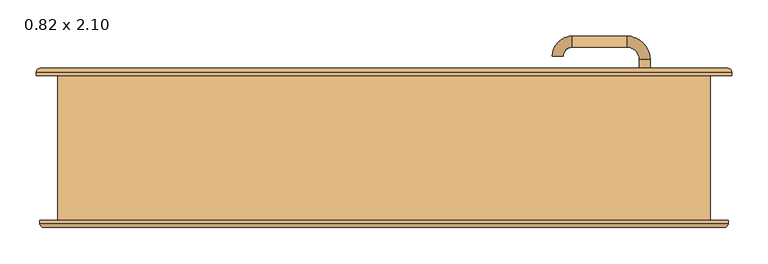
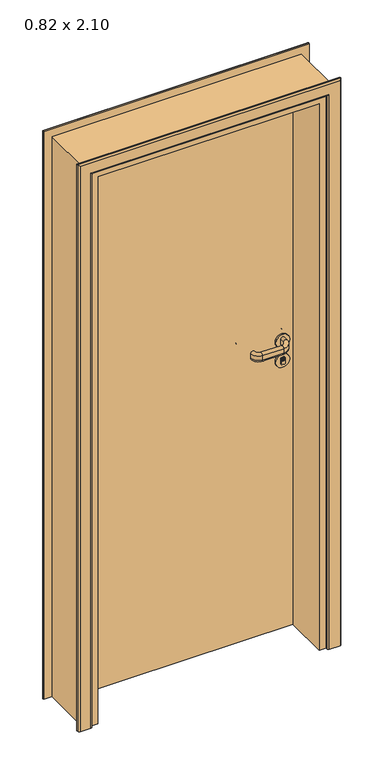
"""IFC4 building model written with IfcOpenShell, lengths in millimetres: door geometry, CC_PORTA ABRIR_1 FOLHA LISA : 0.82 x 2.10."""

from ifc_helpers import new_model, si_unit, point, frame, frame_2d, origin, origin_with_axes, place, context, project, spatial, polyline, circle_curve, ellipse_curve, trimmed, segment, composite_curve, outline, extrude, faceted_brep, source, transform, mapped, element, save
from ifc_brep_helpers import plane_surface, cylinder_surface, revolved_surface, advanced_brep


def door_0_82_x_2_10_06cf7ed5(model_context):
    return source(origin(), model_context, "Body", "SolidModel", [
        advanced_brep(
        [(352.5, 65.0, 1091.5062746), (352.5, 65.0, 1108.3826844), (367.5, 65.0, 1108.3826844), (367.5, 65.0, 1091.5062746), (367.5, 43.0, 1108.3826844), (367.5, 43.0, 1091.5062746), (352.5, 43.0, 1091.5062746), (352.5, 43.0, 1108.3826844), (335.0, 10.5, 1108.3826844), (260.0, 10.5, 1108.3826844), (260.0, 10.5, 1091.5062746), (335.0, 10.5, 1091.5062746), (335.0, 25.5, 1091.5062746), (260.0, 25.5, 1091.5062746), (260.0, 25.5, 1108.3826844), (335.0, 25.5, 1108.3826844), (247.5, 38.0, 1091.5062746), (232.5, 38.0, 1091.5062746), (232.5, 38.0, 1108.3826844), (247.5, 38.0, 1108.3826844)],
        [
            (0, 1),
            (1, 2, circle_curve(frame((360.0, 65.0, 1108.3826844), z_axis=(0.0, 1.0, 0.0), x_axis=(0.0, 0.0, 1.0)), 7.5)),
            (2, 3),
            (3, 0, circle_curve(frame((360.0, 65.0, 1091.5062746), z_axis=(0.0, 1.0, 0.0), x_axis=(0.0, 0.0, 1.0)), 7.5)),
            (2, 4),
            (4, 5),
            (5, 3),
            (0, 6),
            (6, 7),
            (7, 1),
            (8, 9),
            (9, 10),
            (10, 11),
            (11, 8),
            (12, 13),
            (13, 14),
            (14, 15),
            (15, 12),
            (5, 6, circle_curve(frame((360.0, 43.0, 1091.5062746), z_axis=(0.0, 1.0, 0.0), x_axis=(0.0, 0.0, 1.0)), 7.5)),
            (7, 4, circle_curve(frame((360.0, 43.0, 1108.3826844), z_axis=(0.0, 1.0, 0.0), x_axis=(0.0, 0.0, 1.0)), 7.5)),
            (10, 13, circle_curve(frame((260.0, 18.0, 1091.5062746), z_axis=(1.0, 0.0, 0.0), x_axis=(0.0, 0.0, 1.0)), 7.5)),
            (12, 11, circle_curve(frame((335.0, 18.0, 1091.5062746), z_axis=(-1.0, 0.0, 0.0), x_axis=(0.0, 0.0, 1.0)), 7.5)),
            (14, 9, circle_curve(frame((260.0, 18.0, 1108.3826844), z_axis=(1.0, 0.0, 0.0), x_axis=(0.0, 0.0, 1.0)), 7.5)),
            (8, 15, circle_curve(frame((335.0, 18.0, 1108.3826844), z_axis=(-1.0, 0.0, 0.0), x_axis=(0.0, 0.0, 1.0)), 7.5)),
            (12, 6, circle_curve(frame((335.0, 43.0, 1091.5062746), z_axis=(0.0, 0.0, 1.0), x_axis=(1.0, 0.0, 0.0)), 17.5)),
            (5, 11, circle_curve(frame((335.0, 43.0, 1091.5062746), z_axis=(0.0, 0.0, -1.0), x_axis=(1.0, 0.0, 0.0)), 32.5)),
            (4, 8, circle_curve(frame((335.0, 43.0, 1108.3826844), z_axis=(0.0, 0.0, -1.0), x_axis=(1.0, 0.0, 0.0)), 32.5)),
            (7, 15, circle_curve(frame((335.0, 43.0, 1108.3826844), z_axis=(0.0, 0.0, -1.0), x_axis=(1.0, 0.0, 0.0)), 17.5)),
            (16, 17, circle_curve(frame((240.0, 38.0, 1091.5062746), z_axis=(0.0, 1.0, 0.0), x_axis=(0.0, 0.0, 1.0)), 7.5)),
            (17, 18),
            (18, 19, circle_curve(frame((240.0, 38.0, 1108.3826844), z_axis=(0.0, 1.0, 0.0), x_axis=(0.0, 0.0, 1.0)), 7.5)),
            (19, 16),
            (16, 13, circle_curve(frame((260.0, 38.0, 1091.5062746), z_axis=(0.0, 0.0, 1.0), x_axis=(0.0, -1.0, 0.0)), 12.5)),
            (10, 17, circle_curve(frame((260.0, 38.0, 1091.5062746), z_axis=(0.0, 0.0, -1.0), x_axis=(0.0, -1.0, 0.0)), 27.5)),
            (9, 18, circle_curve(frame((260.0, 38.0, 1108.3826844), z_axis=(0.0, 0.0, -1.0), x_axis=(0.0, -1.0, 0.0)), 27.5)),
            (14, 19, circle_curve(frame((260.0, 38.0, 1108.3826844), z_axis=(0.0, 0.0, -1.0), x_axis=(0.0, -1.0, 0.0)), 12.5)),
        ],
        [
            plane_surface(frame((360.0, 65.0, 1099.9444795), z_axis=(0.0, 1.0, 0.0), x_axis=(0.0, 0.0, 1.0))),
            plane_surface(frame((367.5, 65.0, 1091.5062746), z_axis=(1.0, 0.0, 0.0), x_axis=(0.0, -1.0, 0.0))),
            plane_surface(frame((352.5, 65.0, 1108.3826844), z_axis=(-1.0, 0.0, 0.0), x_axis=(0.0, -1.0, 0.0))),
            plane_surface(frame((335.0, 10.5, 1091.5062746), z_axis=(0.0, -1.0, 0.0), x_axis=(-1.0, 0.0, 0.0))),
            plane_surface(frame((335.0, 25.5, 1108.3826844), z_axis=(0.0, 1.0, 0.0), x_axis=(-1.0, 0.0, 0.0))),
            cylinder_surface(frame((360.0, 65.0, 1091.5062746), z_axis=(0.0, 1.0, 0.0), x_axis=(0.0, 0.0, 1.0)), 7.5),
            cylinder_surface(frame((360.0, 65.0, 1108.3826844), z_axis=(0.0, 1.0, 0.0), x_axis=(0.0, 0.0, 1.0)), 7.5),
            cylinder_surface(frame((335.0, 18.0, 1091.5062746), z_axis=(1.0, 0.0, 0.0), x_axis=(0.0, 0.0, 1.0)), 7.5),
            cylinder_surface(frame((335.0, 18.0, 1108.3826844), z_axis=(1.0, 0.0, 0.0), x_axis=(0.0, 0.0, 1.0)), 7.5),
            revolved_surface(trimmed(ellipse_curve(frame((360.0, 43.0, 1091.5062746), z_axis=(0.0, -1.0, 0.0), x_axis=(0.0, 0.0, 1.0)), 7.5, 7.5), [point((352.5, 43.0, 1091.5062746))], [point((367.5, 43.0, 1091.5062746))], True, "CARTESIAN"), (335.0, 43.0, 1099.9444795), (0.0, 0.0, 1.0)),
            cylinder_surface(frame((335.0, 43.0, 1099.9444795), z_axis=(0.0, 0.0, 1.0), x_axis=(1.0, 0.0, 0.0)), 32.5),
            revolved_surface(trimmed(ellipse_curve(frame((360.0, 43.0, 1108.3826844), z_axis=(0.0, -1.0, 0.0), x_axis=(0.0, 0.0, 1.0)), 7.5, 7.5), [point((367.5, 43.0, 1108.3826844))], [point((352.5, 43.0, 1108.3826844))], True, "CARTESIAN"), (335.0, 43.0, 1099.9444795), (0.0, 0.0, 1.0)),
            revolved_surface(polyline([(352.5, 43.0, 1108.3826844), (352.5, 43.0, 1091.5062746)]), (335.0, 43.0, 1099.9444795), (0.0, 0.0, 1.0)),
            plane_surface(frame((240.0, 38.0, 1099.9444795), z_axis=(0.0, 1.0, 0.0), x_axis=(0.0, 0.0, 1.0))),
            revolved_surface(trimmed(ellipse_curve(frame((260.0, 18.0, 1091.5062746), z_axis=(-1.0, 0.0, 0.0), x_axis=(0.0, 0.0, 1.0)), 7.5, 7.5), [point((260.0, 25.5, 1091.5062746))], [point((260.0, 10.5, 1091.5062746))], True, "CARTESIAN"), (260.0, 38.0, 1099.9444795), (0.0, 0.0, 1.0)),
            cylinder_surface(frame((260.0, 38.0, 1099.9444795), z_axis=(0.0, 0.0, 1.0), x_axis=(0.0, -1.0, 0.0)), 27.5),
            revolved_surface(trimmed(ellipse_curve(frame((260.0, 18.0, 1108.3826844), z_axis=(-1.0, 0.0, 0.0), x_axis=(0.0, 0.0, 1.0)), 7.5, 7.5), [point((260.0, 10.5, 1108.3826844))], [point((260.0, 25.5, 1108.3826844))], True, "CARTESIAN"), (260.0, 38.0, 1099.9444795), (0.0, 0.0, 1.0)),
            revolved_surface(polyline([(260.0, 25.5, 1108.3826844), (260.0, 25.5, 1091.5062746)]), (260.0, 38.0, 1099.9444795), (0.0, 0.0, 1.0)),
        ],
        [
            (0, [[1, 2, 3, 4]]),
            (1, [[5, 6, 7, -3]]),
            (2, [[8, 9, 10, -1]]),
            (3, [[11, 12, 13, 14]]),
            (4, [[15, 16, 17, 18]]),
            (5, [[-7, 19, -8, -4]]),
            (6, [[-10, 20, -5, -2]]),
            (7, [[-13, 21, -15, 22]]),
            (8, [[-17, 23, -11, 24]]),
            (9, [[-22, 25, -19, 26]]),
            (10, [[-14, -26, -6, 27]]),
            (11, [[-24, -27, -20, 28]]),
            (12, [[-18, -28, -9, -25]]),
            (13, [[29, 30, 31, 32]]),
            (14, [[-29, 33, -21, 34]]),
            (15, [[-30, -34, -12, 35]]),
            (16, [[-31, -35, -23, 36]]),
            (17, [[-32, -36, -16, -33]]),
        ],
    ),
        extrude(outline(polyline([(361.0, 65.0), (361.0, 55.9), (359.0, 55.9), (359.0, 65.0), (361.0, 65.0)])), frame((0.0, 0.0, 1027.9555433), z_axis=(0.0, 0.0, 1.0), x_axis=(1.0, 0.0, 0.0)), (0.0, 0.0, 1.0), 7.8071257),
        extrude(outline(composite_curve([segment(trimmed(circle_curve(frame_2d((1031.5611613, 360.0)), 5.0), [point((1036.5611613, 360.0))], [point((1026.5611613, 360.0))], False, "CARTESIAN"), True, "CONTINUOUS"), segment(trimmed(circle_curve(frame_2d((1031.5611613, 360.0)), 5.0), [point((1026.5611613, 360.0))], [point((1036.5611613, 360.0))], False, "CARTESIAN"), True, "CONTINUOUS")], self_intersect=False), holes=[polyline([(1035.7626689, 361.0), (1027.9555433, 361.0), (1027.9555433, 359.0), (1035.7626689, 359.0), (1035.7626689, 361.0)])]), frame((0.0, 55.0, 0.0), z_axis=(0.0, 1.0, 0.0), x_axis=(0.0, 0.0, 1.0)), (0.0, 0.0, 1.0), 10.0),
        extrude(outline(composite_curve([segment(polyline([(1033.4817325, 352.5), (1016.4817325, 352.5)]), True, "CONTINUOUS"), segment(trimmed(circle_curve(frame_2d((1016.4817325, 356.5)), 4.0), [point((1016.4817325, 352.5))], [point((1012.4817325, 356.5))], False, "CARTESIAN"), True, "CONTINUOUS"), segment(polyline([(1012.4817325, 356.5), (1012.4817325, 363.5)]), True, "CONTINUOUS"), segment(trimmed(circle_curve(frame_2d((1016.4817325, 363.5)), 4.0), [point((1012.4817325, 363.5))], [point((1016.4817325, 367.5))], False, "CARTESIAN"), True, "CONTINUOUS"), segment(polyline([(1016.4817325, 367.5), (1033.4817325, 367.5)]), True, "CONTINUOUS"), segment(trimmed(circle_curve(frame_2d((1033.4817325, 363.5)), 4.0), [point((1033.4817325, 367.5))], [point((1037.4817325, 363.5))], False, "CARTESIAN"), True, "CONTINUOUS"), segment(polyline([(1037.4817325, 363.5), (1037.4817325, 356.5)]), True, "CONTINUOUS"), segment(trimmed(circle_curve(frame_2d((1033.4817325, 356.5)), 4.0), [point((1037.4817325, 356.5))], [point((1033.4817325, 352.5))], False, "CARTESIAN"), True, "CONTINUOUS")], self_intersect=False)), frame((0.0, 56.0, 0.0), z_axis=(0.0, 1.0, 0.0), x_axis=(0.0, 0.0, 1.0)), (0.0, 0.0, 1.0), 9.0),
        extrude(outline(composite_curve([segment(trimmed(circle_curve(frame_2d((1099.9444795, 360.0)), 25.0), [point((1124.9444795, 360.0))], [point((1074.9444795, 360.0))], False, "CARTESIAN"), True, "CONTINUOUS"), segment(trimmed(circle_curve(frame_2d((1099.9444795, 360.0)), 25.0), [point((1074.9444795, 360.0))], [point((1124.9444795, 360.0))], False, "CARTESIAN"), True, "CONTINUOUS")], self_intersect=False)), frame((0.0, 59.0, 0.0), z_axis=(0.0, 1.0, 0.0), x_axis=(0.0, 0.0, 1.0)), (0.0, 0.0, 1.0), 6.0),
        extrude(outline(composite_curve([segment(trimmed(circle_curve(frame_2d((1024.9444795, 360.0)), 25.0), [point((1049.9444795, 360.0))], [point((999.9444795, 360.0))], False, "CARTESIAN"), True, "CONTINUOUS"), segment(trimmed(circle_curve(frame_2d((1024.9444795, 360.0)), 25.0), [point((999.9444795, 360.0))], [point((1049.9444795, 360.0))], False, "CARTESIAN"), True, "CONTINUOUS")], self_intersect=False), holes=[composite_curve([segment(trimmed(circle_curve(frame_2d((1033.4817325, 363.5)), 4.0), [point((1037.4817325, 363.5))], [point((1033.4817325, 367.5))], True, "CARTESIAN"), True, "CONTINUOUS"), segment(polyline([(1033.4817325, 367.5), (1016.4817325, 367.5)]), True, "CONTINUOUS"), segment(trimmed(circle_curve(frame_2d((1016.4817325, 363.5)), 4.0), [point((1016.4817325, 367.5))], [point((1012.4817325, 363.5))], True, "CARTESIAN"), True, "CONTINUOUS"), segment(polyline([(1012.4817325, 363.5), (1012.4817325, 356.5)]), True, "CONTINUOUS"), segment(trimmed(circle_curve(frame_2d((1016.4817325, 356.5)), 4.0), [point((1012.4817325, 356.5))], [point((1016.4817325, 352.5))], True, "CARTESIAN"), True, "CONTINUOUS"), segment(polyline([(1016.4817325, 352.5), (1033.4817325, 352.5)]), True, "CONTINUOUS"), segment(trimmed(circle_curve(frame_2d((1033.4817325, 356.5)), 4.0), [point((1033.4817325, 352.5))], [point((1037.4817325, 356.5))], True, "CARTESIAN"), True, "CONTINUOUS"), segment(polyline([(1037.4817325, 356.5), (1037.4817325, 363.5)]), True, "CONTINUOUS")], self_intersect=False)]), frame((0.0, 59.0, 0.0), z_axis=(0.0, 1.0, 0.0), x_axis=(0.0, 0.0, 1.0)), (0.0, 0.0, 1.0), 6.0),
        extrude(outline(polyline([(361.0, 109.1), (361.0, 100.0), (359.0, 100.0), (359.0, 109.1), (361.0, 109.1)])), frame((0.0, 0.0, 1027.9555433), z_axis=(0.0, 0.0, 1.0), x_axis=(1.0, 0.0, 0.0)), (0.0, 0.0, 1.0), 7.8071257),
        advanced_brep(
        [(360.0, 110.0, 1036.5611613), (360.0, 110.0, 1026.5611613), (361.0, 110.0, 1035.7626689), (359.0, 110.0, 1035.7626689), (359.0, 110.0, 1027.9555433), (361.0, 110.0, 1027.9555433), (360.0, 100.0, 1049.9444795), (360.0, 100.0, 999.9444795), (360.0, 109.0, 1026.5611613), (360.0, 109.0, 1036.5611613), (361.0, 109.0, 1027.9555433), (361.0, 109.0, 1035.7626689), (359.0, 109.0, 1027.9555433), (359.0, 109.0, 1035.7626689), (352.5, 109.0, 1033.4817325), (356.5, 109.0, 1037.4817325), (363.5, 109.0, 1037.4817325), (367.5, 109.0, 1033.4817325), (367.5, 109.0, 1016.4817325), (363.5, 109.0, 1012.4817325), (356.5, 109.0, 1012.4817325), (352.5, 109.0, 1016.4817325), (352.5, 106.0, 1016.4817325), (352.5, 106.0, 1033.4817325), (356.5, 106.0, 1012.4817325), (363.5, 106.0, 1012.4817325), (367.5, 106.0, 1016.4817325), (367.5, 106.0, 1033.4817325), (363.5, 106.0, 1037.4817325), (356.5, 106.0, 1037.4817325), (360.0, 106.0, 1049.9444795), (360.0, 106.0, 999.9444795)],
        [
            (0, 1, circle_curve(frame((360.0, 110.0, 1031.5611613), z_axis=(0.0, 1.0, 0.0), x_axis=(0.0, 0.0, -1.0)), 5.0)),
            (1, 0, circle_curve(frame((360.0, 110.0, 1031.5611613), z_axis=(0.0, 1.0, 0.0), x_axis=(0.0, 0.0, -1.0)), 5.0)),
            (2, 3),
            (3, 4),
            (4, 5),
            (5, 2),
            (6, 7, circle_curve(frame((360.0, 100.0, 1024.9444795), z_axis=(0.0, -1.0, 0.0), x_axis=(0.0, 0.0, -1.0)), 25.0)),
            (7, 6, circle_curve(frame((360.0, 100.0, 1024.9444795), z_axis=(0.0, -1.0, 0.0), x_axis=(0.0, 0.0, -1.0)), 25.0)),
            (1, 8),
            (8, 9, circle_curve(frame((360.0, 109.0, 1031.5611613), z_axis=(0.0, 1.0, 0.0), x_axis=(0.0, 0.0, -1.0)), 5.0)),
            (9, 0),
            (9, 8, circle_curve(frame((360.0, 109.0, 1031.5611613), z_axis=(0.0, 1.0, 0.0), x_axis=(0.0, 0.0, -1.0)), 5.0)),
            (5, 10),
            (10, 11),
            (11, 2),
            (4, 12),
            (12, 10),
            (3, 13),
            (13, 12),
            (11, 13),
            (14, 15, circle_curve(frame((356.5, 109.0, 1033.4817325), z_axis=(0.0, 1.0, 0.0), x_axis=(0.0, 0.0, -1.0)), 4.0)),
            (15, 16),
            (16, 17, circle_curve(frame((363.5, 109.0, 1033.4817325), z_axis=(0.0, 1.0, 0.0), x_axis=(0.0, 0.0, -1.0)), 4.0)),
            (17, 18),
            (18, 19, circle_curve(frame((363.5, 109.0, 1016.4817325), z_axis=(0.0, 1.0, 0.0), x_axis=(0.0, 0.0, -1.0)), 4.0)),
            (19, 20),
            (20, 21, circle_curve(frame((356.5, 109.0, 1016.4817325), z_axis=(0.0, 1.0, 0.0), x_axis=(0.0, 0.0, -1.0)), 4.0)),
            (21, 14),
            (21, 22),
            (22, 23),
            (23, 14),
            (20, 24),
            (24, 22, circle_curve(frame((356.5, 106.0, 1016.4817325), z_axis=(0.0, 1.0, 0.0), x_axis=(0.0, 0.0, -1.0)), 4.0)),
            (19, 25),
            (25, 24),
            (18, 26),
            (26, 25, circle_curve(frame((363.5, 106.0, 1016.4817325), z_axis=(0.0, 1.0, 0.0), x_axis=(0.0, 0.0, -1.0)), 4.0)),
            (17, 27),
            (27, 26),
            (16, 28),
            (28, 27, circle_curve(frame((363.5, 106.0, 1033.4817325), z_axis=(0.0, 1.0, 0.0), x_axis=(0.0, 0.0, -1.0)), 4.0)),
            (15, 29),
            (29, 28),
            (23, 29, circle_curve(frame((356.5, 106.0, 1033.4817325), z_axis=(0.0, 1.0, 0.0), x_axis=(0.0, 0.0, -1.0)), 4.0)),
            (30, 31, circle_curve(frame((360.0, 106.0, 1024.9444795), z_axis=(0.0, 1.0, 0.0), x_axis=(0.0, 0.0, -1.0)), 25.0)),
            (31, 30, circle_curve(frame((360.0, 106.0, 1024.9444795), z_axis=(0.0, 1.0, 0.0), x_axis=(0.0, 0.0, -1.0)), 25.0)),
            (31, 7),
            (6, 30),
        ],
        [
            plane_surface(frame((360.0, 110.0, 1026.5611613), z_axis=(0.0, 1.0, 0.0), x_axis=(1.0, 0.0, 0.0))),
            plane_surface(frame((360.0, 100.0, 1026.5611613), z_axis=(0.0, -1.0, 0.0), x_axis=(-1.0, 0.0, 0.0))),
            cylinder_surface(frame((360.0, 100.0, 1031.5611613), z_axis=(0.0, 1.0, 0.0), x_axis=(0.0, 0.0, -1.0)), 5.0),
            plane_surface(frame((361.0, 110.0, 1035.7626689), z_axis=(-1.0, 0.0, 0.0), x_axis=(0.0, -1.0, 0.0))),
            plane_surface(frame((361.0, 110.0, 1027.9555433), z_axis=(0.0, 0.0, 1.0), x_axis=(0.0, -1.0, 0.0))),
            plane_surface(frame((359.0, 110.0, 1027.9555433), z_axis=(1.0, 0.0, 0.0), x_axis=(0.0, -1.0, 0.0))),
            plane_surface(frame((359.0, 110.0, 1035.7626689), z_axis=(0.0, 0.0, -1.0), x_axis=(0.0, -1.0, 0.0))),
            plane_surface(frame((352.5, 109.0, 1016.4817325), z_axis=(0.0, 1.0, 0.0), x_axis=(0.0, 0.0, -1.0))),
            plane_surface(frame((352.5, 109.0, 1033.4817325), z_axis=(-1.0, 0.0, 0.0), x_axis=(0.0, -1.0, 0.0))),
            cylinder_surface(frame((356.5, 100.0, 1016.4817325), z_axis=(0.0, 1.0, 0.0), x_axis=(0.0, 0.0, -1.0)), 4.0),
            plane_surface(frame((356.5, 109.0, 1012.4817325), z_axis=(0.0, 0.0, -1.0), x_axis=(0.0, -1.0, 0.0))),
            cylinder_surface(frame((363.5, 100.0, 1016.4817325), z_axis=(0.0, 1.0, 0.0), x_axis=(0.0, 0.0, -1.0)), 4.0),
            plane_surface(frame((367.5, 109.0, 1016.4817325), z_axis=(1.0, 0.0, 0.0), x_axis=(0.0, -1.0, 0.0))),
            cylinder_surface(frame((363.5, 100.0, 1033.4817325), z_axis=(0.0, 1.0, 0.0), x_axis=(0.0, 0.0, -1.0)), 4.0),
            plane_surface(frame((363.5, 109.0, 1037.4817325), z_axis=(0.0, 0.0, 1.0), x_axis=(0.0, -1.0, 0.0))),
            cylinder_surface(frame((356.5, 100.0, 1033.4817325), z_axis=(0.0, 1.0, 0.0), x_axis=(0.0, 0.0, -1.0)), 4.0),
            plane_surface(frame((360.0, 106.0, 1074.9444795), z_axis=(0.0, 1.0, 0.0), x_axis=(1.0, 0.0, 0.0))),
            cylinder_surface(frame((360.0, 100.0, 1024.9444795), z_axis=(0.0, 1.0, 0.0), x_axis=(0.0, 0.0, -1.0)), 25.0),
        ],
        [
            (0, [[1, 2], [3, 4, 5, 6]]),
            (1, [[7, 8]]),
            (2, [[9, 10, 11, -2]]),
            (2, [[-11, 12, -9, -1]]),
            (3, [[13, 14, 15, -6]]),
            (4, [[16, 17, -13, -5]]),
            (5, [[18, 19, -16, -4]]),
            (6, [[-15, 20, -18, -3]]),
            (7, [[-17, -19, -20, -14]]),
            (7, [[21, 22, 23, 24, 25, 26, 27, 28], [-12, -10]]),
            (8, [[29, 30, 31, -28]]),
            (9, [[32, 33, -29, -27]]),
            (10, [[34, 35, -32, -26]]),
            (11, [[36, 37, -34, -25]]),
            (12, [[38, 39, -36, -24]]),
            (13, [[40, 41, -38, -23]]),
            (14, [[42, 43, -40, -22]]),
            (15, [[-31, 44, -42, -21]]),
            (16, [[45, 46], [-33, -35, -37, -39, -41, -43, -44, -30]]),
            (17, [[47, -7, 48, -46]]),
            (17, [[-48, -8, -47, -45]]),
        ],
    ),
        advanced_brep(
        [(360.0, 100.0, 1124.9444795), (360.0, 100.0, 1074.9444795), (360.0, 106.0, 1124.9444795), (360.0, 106.0, 1074.9444795)],
        [
            (0, 1, circle_curve(frame((360.0, 100.0, 1099.9444795), z_axis=(0.0, -1.0, 0.0), x_axis=(0.0, 0.0, -1.0)), 25.0)),
            (1, 0, circle_curve(frame((360.0, 100.0, 1099.9444795), z_axis=(0.0, -1.0, 0.0), x_axis=(0.0, 0.0, -1.0)), 25.0)),
            (2, 3, circle_curve(frame((360.0, 106.0, 1099.9444795), z_axis=(0.0, 1.0, 0.0), x_axis=(0.0, 0.0, -1.0)), 25.0)),
            (3, 2, circle_curve(frame((360.0, 106.0, 1099.9444795), z_axis=(0.0, 1.0, 0.0), x_axis=(0.0, 0.0, -1.0)), 25.0)),
            (3, 1),
            (0, 2),
        ],
        [
            plane_surface(frame((360.0, 100.0, 1026.5611613), z_axis=(0.0, -1.0, 0.0), x_axis=(-1.0, 0.0, 0.0))),
            plane_surface(frame((360.0, 106.0, 1074.9444795), z_axis=(0.0, 1.0, 0.0), x_axis=(1.0, 0.0, 0.0))),
            cylinder_surface(frame((360.0, 100.0, 1099.9444795), z_axis=(0.0, 1.0, 0.0), x_axis=(0.0, 0.0, -1.0)), 25.0),
        ],
        [
            (0, [[1, 2]]),
            (1, [[3, 4]]),
            (2, [[5, -1, 6, -4]]),
            (2, [[-6, -2, -5, -3]]),
        ],
    ),
        advanced_brep(
        [(352.5, 100.0, 1108.4382049), (352.5, 100.0, 1091.5617951), (367.5, 100.0, 1091.5617951), (367.5, 100.0, 1108.4382049), (367.5, 122.0, 1091.5617951), (367.5, 122.0, 1108.4382049), (352.5, 122.0, 1108.4382049), (352.5, 122.0, 1091.5617951), (335.0, 154.5, 1091.5617951), (260.0, 154.5, 1091.5617951), (260.0, 154.5, 1108.4382049), (335.0, 154.5, 1108.4382049), (335.0, 139.5, 1108.4382049), (260.0, 139.5, 1108.4382049), (260.0, 139.5, 1091.5617951), (335.0, 139.5, 1091.5617951), (247.5, 127.0, 1108.4382049), (232.5, 127.0, 1108.4382049), (232.5, 127.0, 1091.5617951), (247.5, 127.0, 1091.5617951)],
        [
            (0, 1),
            (1, 2, circle_curve(frame((360.0, 100.0, 1091.5617951), z_axis=(0.0, -1.0, 0.0), x_axis=(-1.0, 0.0, 0.0)), 7.5)),
            (2, 3),
            (3, 0, circle_curve(frame((360.0, 100.0, 1108.4382049), z_axis=(0.0, -1.0, 0.0), x_axis=(-1.0, 0.0, 0.0)), 7.5)),
            (2, 4),
            (4, 5),
            (5, 3),
            (0, 6),
            (6, 7),
            (7, 1),
            (8, 9),
            (9, 10),
            (10, 11),
            (11, 8),
            (12, 13),
            (13, 14),
            (14, 15),
            (15, 12),
            (5, 6, circle_curve(frame((360.0, 122.0, 1108.4382049), z_axis=(0.0, -1.0, 0.0), x_axis=(-1.0, 0.0, 0.0)), 7.5)),
            (7, 4, circle_curve(frame((360.0, 122.0, 1091.5617951), z_axis=(0.0, -1.0, 0.0), x_axis=(-1.0, 0.0, 0.0)), 7.5)),
            (10, 13, circle_curve(frame((260.0, 147.0, 1108.4382049), z_axis=(1.0, 0.0, 0.0), x_axis=(0.0, -1.0, 0.0)), 7.5)),
            (12, 11, circle_curve(frame((335.0, 147.0, 1108.4382049), z_axis=(-1.0, 0.0, 0.0), x_axis=(0.0, -1.0, 0.0)), 7.5)),
            (14, 9, circle_curve(frame((260.0, 147.0, 1091.5617951), z_axis=(1.0, 0.0, 0.0), x_axis=(0.0, -1.0, 0.0)), 7.5)),
            (8, 15, circle_curve(frame((335.0, 147.0, 1091.5617951), z_axis=(-1.0, 0.0, 0.0), x_axis=(0.0, -1.0, 0.0)), 7.5)),
            (12, 6, circle_curve(frame((335.0, 122.0, 1108.4382049), z_axis=(0.0, 0.0, -1.0), x_axis=(1.0, 0.0, 0.0)), 17.5)),
            (5, 11, circle_curve(frame((335.0, 122.0, 1108.4382049), z_axis=(0.0, 0.0, 1.0), x_axis=(1.0, 0.0, 0.0)), 32.5)),
            (4, 8, circle_curve(frame((335.0, 122.0, 1091.5617951), z_axis=(0.0, 0.0, 1.0), x_axis=(1.0, 0.0, 0.0)), 32.5)),
            (7, 15, circle_curve(frame((335.0, 122.0, 1091.5617951), z_axis=(0.0, 0.0, 1.0), x_axis=(1.0, 0.0, 0.0)), 17.5)),
            (16, 17, circle_curve(frame((240.0, 127.0, 1108.4382049), z_axis=(0.0, -1.0, 0.0), x_axis=(1.0, 0.0, 0.0)), 7.5)),
            (17, 18),
            (18, 19, circle_curve(frame((240.0, 127.0, 1091.5617951), z_axis=(0.0, -1.0, 0.0), x_axis=(1.0, 0.0, 0.0)), 7.5)),
            (19, 16),
            (16, 13, circle_curve(frame((260.0, 127.0, 1108.4382049), z_axis=(0.0, 0.0, -1.0), x_axis=(0.0, 1.0, 0.0)), 12.5)),
            (10, 17, circle_curve(frame((260.0, 127.0, 1108.4382049), z_axis=(0.0, 0.0, 1.0), x_axis=(0.0, 1.0, 0.0)), 27.5)),
            (9, 18, circle_curve(frame((260.0, 127.0, 1091.5617951), z_axis=(0.0, 0.0, 1.0), x_axis=(0.0, 1.0, 0.0)), 27.5)),
            (14, 19, circle_curve(frame((260.0, 127.0, 1091.5617951), z_axis=(0.0, 0.0, 1.0), x_axis=(0.0, 1.0, 0.0)), 12.5)),
        ],
        [
            plane_surface(frame((360.0, 100.0, 1100.0), z_axis=(0.0, -1.0, 0.0), x_axis=(0.0, 0.0, -1.0))),
            plane_surface(frame((367.5, 100.0, 1108.4382049), z_axis=(1.0, 0.0, 0.0), x_axis=(0.0, 1.0, 0.0))),
            plane_surface(frame((352.5, 100.0, 1091.5617951), z_axis=(-1.0, 0.0, 0.0), x_axis=(0.0, 1.0, 0.0))),
            plane_surface(frame((335.0, 154.5, 1108.4382049), z_axis=(0.0, 1.0, 0.0), x_axis=(-1.0, 0.0, 0.0))),
            plane_surface(frame((335.0, 139.5, 1091.5617951), z_axis=(0.0, -1.0, 0.0), x_axis=(-1.0, 0.0, 0.0))),
            cylinder_surface(frame((360.0, 100.0, 1108.4382049), z_axis=(0.0, -1.0, 0.0), x_axis=(-1.0, 0.0, 0.0)), 7.5),
            cylinder_surface(frame((360.0, 100.0, 1091.5617951), z_axis=(0.0, -1.0, 0.0), x_axis=(-1.0, 0.0, 0.0)), 7.5),
            cylinder_surface(frame((335.0, 147.0, 1108.4382049), z_axis=(1.0, 0.0, 0.0), x_axis=(0.0, -1.0, 0.0)), 7.5),
            cylinder_surface(frame((335.0, 147.0, 1091.5617951), z_axis=(1.0, 0.0, 0.0), x_axis=(0.0, -1.0, 0.0)), 7.5),
            revolved_surface(trimmed(ellipse_curve(frame((360.0, 122.0, 1108.4382049), z_axis=(0.0, 1.0, 0.0), x_axis=(-1.0, 0.0, 0.0)), 7.5, 7.5), [point((352.5, 122.0, 1108.4382049))], [point((367.5, 122.0, 1108.4382049))], True, "CARTESIAN"), (335.0, 122.0, 1100.0), (0.0, 0.0, -1.0)),
            cylinder_surface(frame((335.0, 122.0, 1100.0), z_axis=(0.0, 0.0, -1.0), x_axis=(1.0, 0.0, 0.0)), 32.5),
            revolved_surface(trimmed(ellipse_curve(frame((360.0, 122.0, 1091.5617951), z_axis=(0.0, 1.0, 0.0), x_axis=(-1.0, 0.0, 0.0)), 7.5, 7.5), [point((367.5, 122.0, 1091.5617951))], [point((352.5, 122.0, 1091.5617951))], True, "CARTESIAN"), (335.0, 122.0, 1100.0), (0.0, 0.0, -1.0)),
            revolved_surface(polyline([(352.5, 122.0, 1091.5617951), (352.5, 122.0, 1108.4382049)]), (335.0, 122.0, 1100.0), (0.0, 0.0, -1.0)),
            plane_surface(frame((240.0, 127.0, 1100.0), z_axis=(0.0, -1.0, 0.0), x_axis=(0.0, 0.0, -1.0))),
            revolved_surface(trimmed(ellipse_curve(frame((260.0, 147.0, 1108.4382049), z_axis=(-1.0, 0.0, 0.0), x_axis=(0.0, -1.0, 0.0)), 7.5, 7.5), [point((260.0, 139.5, 1108.4382049))], [point((260.0, 154.5, 1108.4382049))], True, "CARTESIAN"), (260.0, 127.0, 1100.0), (0.0, 0.0, -1.0)),
            cylinder_surface(frame((260.0, 127.0, 1100.0), z_axis=(0.0, 0.0, -1.0), x_axis=(0.0, 1.0, 0.0)), 27.5),
            revolved_surface(trimmed(ellipse_curve(frame((260.0, 147.0, 1091.5617951), z_axis=(-1.0, 0.0, 0.0), x_axis=(0.0, -1.0, 0.0)), 7.5, 7.5), [point((260.0, 154.5, 1091.5617951))], [point((260.0, 139.5, 1091.5617951))], True, "CARTESIAN"), (260.0, 127.0, 1100.0), (0.0, 0.0, -1.0)),
            revolved_surface(polyline([(260.0, 139.5, 1091.5617951), (260.0, 139.5, 1108.4382049)]), (260.0, 127.0, 1100.0), (0.0, 0.0, -1.0)),
        ],
        [
            (0, [[1, 2, 3, 4]]),
            (1, [[5, 6, 7, -3]]),
            (2, [[8, 9, 10, -1]]),
            (3, [[11, 12, 13, 14]]),
            (4, [[15, 16, 17, 18]]),
            (5, [[-7, 19, -8, -4]]),
            (6, [[-10, 20, -5, -2]]),
            (7, [[-13, 21, -15, 22]]),
            (8, [[-17, 23, -11, 24]]),
            (9, [[-22, 25, -19, 26]]),
            (10, [[-14, -26, -6, 27]]),
            (11, [[-24, -27, -20, 28]]),
            (12, [[-18, -28, -9, -25]]),
            (13, [[29, 30, 31, 32]]),
            (14, [[-29, 33, -21, 34]]),
            (15, [[-30, -34, -12, 35]]),
            (16, [[-31, -35, -23, 36]]),
            (17, [[-32, -36, -16, -33]]),
        ],
    ),
        extrude(outline(polyline([(410.0, 100.0), (410.0, 65.0), (-410.0, 65.0), (-410.0, 100.0), (410.0, 100.0)])), origin_with_axes(), (0.0, 0.0, 1.0), 2100.0),
        advanced_brep(
        [(-430.5, -110.0, 0.0), (-469.500573, -110.0, 0.0), (-475.0, -104.500573, 0.0), (-475.0, -100.0, 0.0), (-425.0, -100.0, 0.0), (-425.0, -104.5, 0.0), (-425.0, -104.5, 2115.0), (-430.5, -110.0, 2120.5), (-425.0, -100.0, 2115.0), (-475.0, -100.0, 2165.0), (475.0, -100.0, 2165.0), (475.0, -100.0, 0.0), (425.0, -100.0, 0.0), (425.0, -100.0, 2115.0), (-475.0, -104.500573, 2165.0), (-469.500573, -110.0, 2159.500573), (430.5, -110.0, 2120.5), (430.5, -110.0, 0.0), (469.500573, -110.0, 0.0), (469.500573, -110.0, 2159.500573), (425.0, -104.5, 0.0), (425.0, -104.5, 2115.0), (475.0, -104.500573, 0.0), (475.0, -104.500573, 2165.0)],
        [
            (0, 1),
            (1, 2, circle_curve(frame((-469.500573, -104.500573, 0.0), z_axis=(0.0, 0.0, -1.0), x_axis=(0.0, -1.0, 0.0)), 5.499427)),
            (2, 3),
            (3, 4),
            (4, 5),
            (5, 0, circle_curve(frame((-430.5, -104.5, 0.0), z_axis=(0.0, 0.0, -1.0), x_axis=(0.0, -1.0, 0.0)), 5.5)),
            (5, 6),
            (6, 7, ellipse_curve(frame((-430.5, -104.5, 2120.5), z_axis=(-0.7071067811865475, 0.0, -0.7071067811865475), x_axis=(0.7071067811865474, 0.0, -0.7071067811865476)), 7.7781746, 5.5)),
            (7, 0),
            (4, 8),
            (8, 6),
            (3, 9),
            (9, 10),
            (10, 11),
            (11, 12),
            (12, 13),
            (13, 8),
            (2, 14),
            (14, 9),
            (1, 15),
            (15, 14, ellipse_curve(frame((-469.500573, -104.500573, 2159.500573), z_axis=(-0.7071067811865475, 0.0, -0.7071067811865475), x_axis=(0.7071067811865474, 0.0, -0.7071067811865476)), 7.7773642, 5.499427)),
            (7, 16),
            (16, 17),
            (17, 18),
            (18, 19),
            (19, 15),
            (12, 20),
            (20, 21),
            (21, 13),
            (17, 20, circle_curve(frame((430.5, -104.5, 0.0), z_axis=(0.0, 0.0, -1.0), x_axis=(0.0, -1.0, 0.0)), 5.5)),
            (11, 22),
            (22, 18, circle_curve(frame((469.500573, -104.500573, 0.0), z_axis=(0.0, 0.0, -1.0), x_axis=(0.0, -1.0, 0.0)), 5.499427)),
            (23, 22),
            (10, 23),
            (23, 19, ellipse_curve(frame((469.500573, -104.500573, 2159.500573), z_axis=(0.7071067811865475, 0.0, -0.7071067811865475), x_axis=(0.7071067811865474, 0.0, 0.7071067811865476)), 7.7773642, 5.499427)),
            (16, 21, ellipse_curve(frame((430.5, -104.5, 2120.5), z_axis=(0.7071067811865475, 0.0, -0.7071067811865475), x_axis=(0.7071067811865474, 0.0, 0.7071067811865476)), 7.7781746, 5.5)),
            (6, 21),
            (14, 23),
        ],
        [
            plane_surface(frame((-450.0, -100.0, 0.0), z_axis=(0.0, 0.0, -1.0), x_axis=(-1.0, 0.0, 0.0))),
            cylinder_surface(frame((-430.5, -104.5, 0.0), z_axis=(0.0, 0.0, -1.0), x_axis=(0.0, -1.0, 0.0)), 5.5),
            plane_surface(frame((-425.0, -104.5, 0.0), z_axis=(1.0, 0.0, 0.0), x_axis=(0.0, 0.0, 1.0))),
            plane_surface(frame((-425.0, -100.0, 0.0), z_axis=(0.0, 1.0, 0.0), x_axis=(0.0, 0.0, 1.0))),
            plane_surface(frame((-475.0, -100.0, 0.0), z_axis=(-1.0, 0.0, 0.0), x_axis=(0.0, 0.0, 1.0))),
            cylinder_surface(frame((-469.500573, -104.500573, 0.0), z_axis=(0.0, 0.0, -1.0), x_axis=(0.0, -1.0, 0.0)), 5.499427),
            plane_surface(frame((-469.500573, -110.0, 0.0), z_axis=(0.0, -1.0, 0.0), x_axis=(0.0, 0.0, 1.0))),
            plane_surface(frame((425.0, -104.5, 2115.0), z_axis=(-1.0, 0.0, 0.0), x_axis=(0.0, 0.0, -1.0))),
            plane_surface(frame((450.0, -100.0, 0.0), z_axis=(0.0, 0.0, -1.0), x_axis=(1.0, 0.0, 0.0))),
            plane_surface(frame((475.0, -100.0, 2165.0), z_axis=(1.0, 0.0, 0.0), x_axis=(0.0, 0.0, -1.0))),
            cylinder_surface(frame((469.500573, -104.500573, 2140.0), z_axis=(0.0, 0.0, 1.0), x_axis=(0.0, -1.0, 0.0)), 5.499427),
            cylinder_surface(frame((430.5, -104.5, 2140.0), z_axis=(0.0, 0.0, 1.0), x_axis=(0.0, -1.0, 0.0)), 5.5),
            cylinder_surface(frame((-450.0, -104.5, 2120.5), z_axis=(-1.0, 0.0, 0.0), x_axis=(0.0, -1.0, 0.0)), 5.5),
            plane_surface(frame((-425.0, -104.5, 2115.0), z_axis=(0.0, 0.0, -1.0), x_axis=(1.0, 0.0, 0.0))),
            plane_surface(frame((-475.0, -100.0, 2165.0), z_axis=(0.0, 0.0, 1.0), x_axis=(1.0, 0.0, 0.0))),
            cylinder_surface(frame((-450.0, -104.500573, 2159.500573), z_axis=(-1.0, 0.0, 0.0), x_axis=(0.0, -1.0, 0.0)), 5.499427),
        ],
        [
            (0, [[1, 2, 3, 4, 5, 6]]),
            (1, [[7, 8, 9, -6]]),
            (2, [[10, 11, -7, -5]]),
            (3, [[12, 13, 14, 15, 16, 17, -10, -4]]),
            (4, [[18, 19, -12, -3]]),
            (5, [[20, 21, -18, -2]]),
            (6, [[-9, 22, 23, 24, 25, 26, -20, -1]]),
            (7, [[-16, 27, 28, 29]]),
            (8, [[30, -27, -15, 31, 32, -24]]),
            (9, [[33, -31, -14, 34]]),
            (10, [[-25, -32, -33, 35]]),
            (11, [[-28, -30, -23, 36]]),
            (12, [[37, -36, -22, -8]]),
            (13, [[-17, -29, -37, -11]]),
            (14, [[38, -34, -13, -19]]),
            (15, [[-26, -35, -38, -21]]),
        ],
    ),
        advanced_brep(
        [(-430.0, 100.0, 0.0), (-480.0, 100.0, 0.0), (-480.0, 104.5, 0.0), (-474.5, 110.0, 0.0), (-435.5, 110.0, 0.0), (-430.0, 104.5, 0.0), (-430.0, 104.5, 2120.0), (-430.0, 100.0, 2120.0), (-435.5, 110.0, 2125.5), (-474.5, 110.0, 2164.5), (474.5, 110.0, 2164.5), (474.5, 110.0, 0.0), (435.5, 110.0, 0.0), (435.5, 110.0, 2125.5), (-480.0, 104.5, 2170.0), (-480.0, 100.0, 2170.0), (430.0, 100.0, 2120.0), (430.0, 100.0, 0.0), (480.0, 100.0, 0.0), (480.0, 100.0, 2170.0), (430.0, 104.5, 0.0), (430.0, 104.5, 2120.0), (480.0, 104.5, 0.0), (480.0, 104.5, 2170.0)],
        [
            (0, 1),
            (1, 2),
            (2, 3, circle_curve(frame((-474.5, 104.5, 0.0), z_axis=(0.0, 0.0, -1.0), x_axis=(0.0, -1.0, 0.0)), 5.5)),
            (3, 4),
            (4, 5, circle_curve(frame((-435.5, 104.5, 0.0), z_axis=(0.0, 0.0, -1.0), x_axis=(0.0, -1.0, 0.0)), 5.5)),
            (5, 0),
            (5, 6),
            (6, 7),
            (7, 0),
            (4, 8),
            (8, 6, ellipse_curve(frame((-435.5, 104.5, 2125.5), z_axis=(-0.7071067811865475, 0.0, -0.7071067811865475), x_axis=(0.7071067811865474, 0.0, -0.7071067811865476)), 7.7781746, 5.5)),
            (3, 9),
            (9, 10),
            (10, 11),
            (11, 12),
            (12, 13),
            (13, 8),
            (2, 14),
            (14, 9, ellipse_curve(frame((-474.5, 104.5, 2164.5), z_axis=(-0.7071067811865475, 0.0, -0.7071067811865475), x_axis=(0.7071067811865474, 0.0, -0.7071067811865476)), 7.7781746, 5.5)),
            (1, 15),
            (15, 14),
            (7, 16),
            (16, 17),
            (17, 18),
            (18, 19),
            (19, 15),
            (12, 20, circle_curve(frame((435.5, 104.5, 0.0), z_axis=(0.0, 0.0, 1.0), x_axis=(0.0, -1.0, 0.0)), 5.5)),
            (20, 21),
            (21, 13, ellipse_curve(frame((435.5, 104.5, 2125.5), z_axis=(0.7071067811865475, 0.0, -0.7071067811865475), x_axis=(0.7071067811865474, 0.0, 0.7071067811865476)), 7.7781746, 5.5)),
            (17, 20),
            (11, 22, circle_curve(frame((474.5, 104.5, 0.0), z_axis=(0.0, 0.0, -1.0), x_axis=(0.0, -1.0, 0.0)), 5.5)),
            (22, 18),
            (23, 22),
            (10, 23, ellipse_curve(frame((474.5, 104.5, 2164.5), z_axis=(0.7071067811865475, 0.0, -0.7071067811865475), x_axis=(0.7071067811865474, 0.0, 0.7071067811865476)), 7.7781746, 5.5)),
            (23, 19),
            (16, 21),
            (6, 21),
            (14, 23),
        ],
        [
            plane_surface(frame((-450.0, 100.0, 0.0), z_axis=(0.0, 0.0, -1.0), x_axis=(-1.0, 0.0, 0.0))),
            plane_surface(frame((-430.0, 100.0, 0.0), z_axis=(1.0, 0.0, 0.0), x_axis=(0.0, 0.0, 1.0))),
            cylinder_surface(frame((-435.5, 104.5, 0.0), z_axis=(0.0, 0.0, -1.0), x_axis=(0.0, -1.0, 0.0)), 5.5),
            plane_surface(frame((-435.5, 110.0, 0.0), z_axis=(0.0, 1.0, 0.0), x_axis=(0.0, 0.0, 1.0))),
            cylinder_surface(frame((-474.5, 104.5, 0.0), z_axis=(0.0, 0.0, -1.0), x_axis=(0.0, -1.0, 0.0)), 5.5),
            plane_surface(frame((-480.0, 104.5, 0.0), z_axis=(-1.0, 0.0, 0.0), x_axis=(0.0, 0.0, 1.0))),
            plane_surface(frame((-480.0, 100.0, 0.0), z_axis=(0.0, -1.0, 0.0), x_axis=(0.0, 0.0, 1.0))),
            cylinder_surface(frame((435.5, 104.5, 2140.0), z_axis=(0.0, 0.0, 1.0), x_axis=(0.0, -1.0, 0.0)), 5.5),
            plane_surface(frame((450.0, 100.0, 0.0), z_axis=(0.0, 0.0, -1.0), x_axis=(1.0, 0.0, 0.0))),
            cylinder_surface(frame((474.5, 104.5, 2140.0), z_axis=(0.0, 0.0, 1.0), x_axis=(0.0, -1.0, 0.0)), 5.5),
            plane_surface(frame((480.0, 104.5, 2170.0), z_axis=(1.0, 0.0, 0.0), x_axis=(0.0, 0.0, -1.0))),
            plane_surface(frame((430.0, 100.0, 2120.0), z_axis=(-1.0, 0.0, 0.0), x_axis=(0.0, 0.0, -1.0))),
            plane_surface(frame((-430.0, 100.0, 2120.0), z_axis=(0.0, 0.0, -1.0), x_axis=(1.0, 0.0, 0.0))),
            cylinder_surface(frame((-450.0, 104.5, 2125.5), z_axis=(-1.0, 0.0, 0.0), x_axis=(0.0, -1.0, 0.0)), 5.5),
            cylinder_surface(frame((-450.0, 104.5, 2164.5), z_axis=(-1.0, 0.0, 0.0), x_axis=(0.0, -1.0, 0.0)), 5.5),
            plane_surface(frame((-480.0, 104.5, 2170.0), z_axis=(0.0, 0.0, 1.0), x_axis=(1.0, 0.0, 0.0))),
        ],
        [
            (0, [[1, 2, 3, 4, 5, 6]]),
            (1, [[7, 8, 9, -6]]),
            (2, [[10, 11, -7, -5]]),
            (3, [[12, 13, 14, 15, 16, 17, -10, -4]]),
            (4, [[18, 19, -12, -3]]),
            (5, [[20, 21, -18, -2]]),
            (6, [[-9, 22, 23, 24, 25, 26, -20, -1]]),
            (7, [[-16, 27, 28, 29]]),
            (8, [[30, -27, -15, 31, 32, -24]]),
            (9, [[33, -31, -14, 34]]),
            (10, [[-25, -32, -33, 35]]),
            (11, [[-28, -30, -23, 36]]),
            (12, [[37, -36, -22, -8]]),
            (13, [[-17, -29, -37, -11]]),
            (14, [[38, -34, -13, -19]]),
            (15, [[-26, -35, -38, -21]]),
        ],
    ),
        faceted_brep([(-410.0, 65.0, 0.0), (-400.0, 65.0, 0.0), (-400.0, -100.0, 0.0), (-450.0, -100.0, 0.0), (-450.0, 100.0, 0.0), (-410.0, 100.0, 0.0), (-410.0, 100.0, 2100.0), (-410.0, 65.0, 2100.0), (-450.0, 100.0, 2140.0), (450.0, 100.0, 2140.0), (450.0, 100.0, 0.0), (410.0, 100.0, 0.0), (410.0, 100.0, 2100.0), (-450.0, -100.0, 2140.0), (-400.0, -100.0, 2090.0), (400.0, -100.0, 2090.0), (400.0, -100.0, 0.0), (450.0, -100.0, 0.0), (450.0, -100.0, 2140.0), (-400.0, 65.0, 2090.0), (410.0, 65.0, 2100.0), (410.0, 65.0, 0.0), (400.0, 65.0, 0.0), (400.0, 65.0, 2090.0)], [[[0, 1, 2, 3, 4, 5]], [[5, 6, 7, 0]], [[4, 8, 9, 10, 11, 12, 6, 5]], [[3, 13, 8, 4]], [[2, 14, 15, 16, 17, 18, 13, 3]], [[1, 19, 14, 2]], [[0, 7, 20, 21, 22, 23, 19, 1]], [[12, 11, 21, 20]], [[21, 11, 10, 17, 16, 22]], [[18, 17, 10, 9]], [[23, 22, 16, 15]], [[6, 12, 20, 7]], [[13, 18, 9, 8]], [[19, 23, 15, 14]]]),
    ])


if __name__ == "__main__":
    model = new_model("IFC4")
    model_context = context("Model", 3, world=origin())
    ifc_project = project(units=[si_unit("LENGTHUNIT", "METRE", prefix="MILLI")], contexts=[model_context])
    site = spatial("IfcSite", under=ifc_project)
    building = spatial("IfcBuilding", under=site)
    placement = place(None, origin())
    door_0_82_x_2_10_shape = door_0_82_x_2_10_06cf7ed5(model_context)
    element("IfcDoor", 1, ObjectType="CC_PORTA ABRIR_1 FOLHA LISA : 0.82 x 2.10", at=placement, inside=building, context=model_context, shape_type="MappedRepresentation", body=[
        mapped(door_0_82_x_2_10_shape, transform((0.0, 0.0, 0.0), x_axis=(1.0, 0.0, 0.0), y_axis=(0.0, 1.0, 0.0), z_axis=(0.0, 0.0, 1.0))),
    ])
    save(model, "model.ifc")

# Revit data of these elements
# Type "CC_PORTA ABRIR_1 FOLHA LISA : 0.82 x 2.10"
#   Type Mark = "P2"
#   Site = "www.construir.arq.br"
#   Empresa = "Cursos Construir"
#   Description = "PORTA ABRIR 1 FOLHA LISA"
#   Criado Por = "Roberto Netto"
#   Analytic Construction = "<Nenhum>"
#   Atualizado por = "Rudemberg Eloi"
#   Rough Width = 0.90 m
#   Interna [instance default] = 0.00 m
#   Largura Guarnição Interna [instance default] = 0.05 m
#   Largura Guarnição Externa [instance default] = 0.05 m
#   Largura Folha [instance default] = 0.82 m
#   Externa [instance default] = 0.00 m
#   Extensão Lateral Esquerda [instance default] = 0.03 m
#   Extensão Lateral Direita [instance default] = 0.03 m
#   Extensão Frontal [instance default] = 0.03 m
#   Espessura Soleira [instance default] = 0.02 m
#   Espessura Guarnição Interna [instance default] = 0.01 m
#   Espessura Guarnição Externa [instance default] = 0.01 m
#   Espessura Folha [instance default] = 0.035 m
#   Espessura Batente [instance default] = 0.05 m
#   Eixo Rotação Folha [instance default] = 0.04 m
#   Deslocamento Maçaneta [instance default] = 0.05 m
#   Deslocamento Fechadura [instance default] = 0.05 m
#   Desloc (Interno) [instance default] = 0.02 m
#   Desloc (Externo) [instance default] = 0.025 m
#   Rough Height = 2.14 m
#   Altura Maçaneta [instance default] = 1.10 m
#   Altura Folha [instance default] = 2.10 m
#   Altura Fechadura [instance default] = 1.00 m
#   Height = 2.14 m
#   Width = 0.90 m
#   ----SOLEIRA---- [instance default] = 0.00 m
#   ----MAÇANETA/FECHADURA---- [instance default] = 0.00 m
#   ----GUARNIÇÃO---- [instance default] = 0.00 m
#   ----FOLHA---- [instance default] = 0.00 m
#   ----EXTENSÃO---- [instance default] = 0.00 m
#   ----BATENTE---- [instance default] = 0.00 m
#   Soleira Sem Extensão [instance default] = yes
#   Soleira Com Extensão [instance default] = no
#   Soleira [instance default] = yes
#   Maçaneta / Puxador [instance default] = yes
#   Guarnição Interna [instance default] = yes
#   Guarnição Externa [instance default] = yes
#   Fechadura Separada [instance default] = no
#   Bit [instance default] = no
#   Porcent. Exibição Batente Interno [instance default] = 50
#   Porcent. Exibição Batente Externo [instance default] = 50
#   Material Bit/Soleira = .GRANITO BRANCO ITAÚNAS
#   Material Espelho/Fixação = .AÇO INOXIDÁVEL ESCOVADO
#   Material Maçaneta/Puxador = .AÇO INOXIDÁVEL ESCOVADO
#   Material Guarnição Interna = .MADEIRA COM PINTURA ESMALTE BRANCO ACETINADO
#   Material Guarnição Externa = .MADEIRA COM PINTURA ESMALTE BRANCO ACETINADO
#   Material Folha = .MADEIRA COM PINTURA ESMALTE BRANCO ACETINADO
#   Material Fechadura = .AÇO INOXIDÁVEL ESCOVADO
#   Material Batente = .MADEIRA COM PINTURA ESMALTE BRANCO ACETINADO
#   Família Maçaneta [instance default] = element 613477
#   Function = (empty or 0)
#   Wall Closure = (empty or 0)
# Element 1 (IfcDoor, "CC_PORTA ABRIR_1 FOLHA LISA : 0.82 x 2.10")
#   Materials on its faces: ".AÇO INOXIDÁVEL ESCOVADO", ".MADEIRA COM PINTURA ESMALTE BRANCO ACETINADO"
# Materials
#   ".GRANITO BRANCO ITAÚNAS": class ".CC_PEDRA REVEST.", colour RGB 202 195 174, transparency 0, Description = "Granito branco Itaúnas", Uso = "Pedra", Cost = 0
#   ".AÇO INOXIDÁVEL ESCOVADO": class "Metal", colour RGB 189 187 185, transparency 0, Description = "Stainless Steel 18/8, brushed finish", Cost = 0
#   ".MADEIRA COM PINTURA ESMALTE BRANCO ACETINADO": class ".CC_MADEIRAS", colour RGB 240 240 240, transparency 0, Description = "Madeira com pintura esmalte branco acetinado.", Cost = 0
